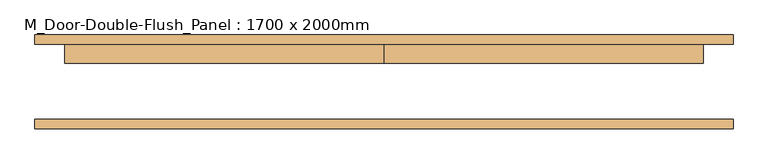
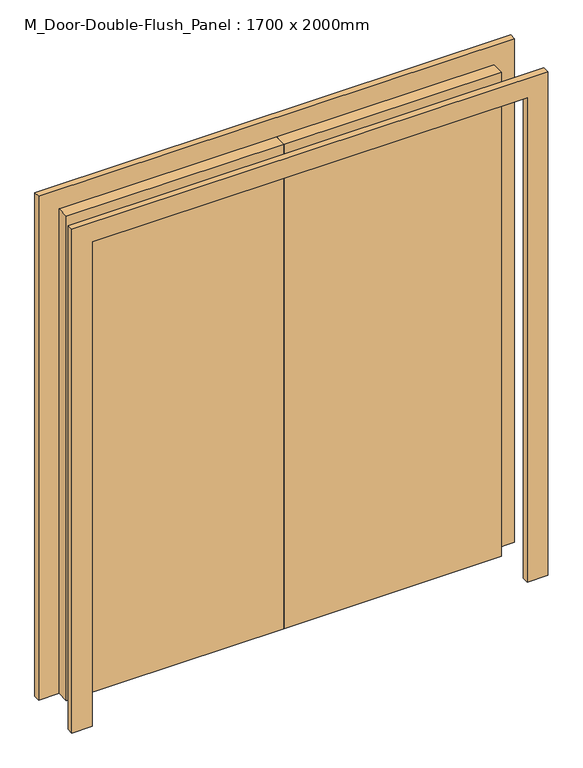
"""IFC4 building model written with IfcOpenShell, lengths in millimetres: door geometry, M_Door-Double-Flush_Panel : 1700 x 2000mm."""

from ifc_helpers import new_model, si_unit, frame, origin, origin_with_axes, place, context, project, spatial, polyline, outline, extrude, source, transform, mapped, element, save


def m_door_double_flush_panel_1700_x_2000mm_deeb3825(model_context):
    return source(origin(), model_context, "Body", "SweptSolid", [
        extrude(outline(polyline([(2000.0, -850.0), (2000.0, 850.0), (0.0, 850.0), (0.0, 930.0), (2080.0, 930.0), (2080.0, -930.0), (0.0, -930.0), (0.0, -850.0), (2000.0, -850.0)])), frame((0.0, -125.0, 0.0), z_axis=(0.0, 1.0, 0.0), x_axis=(0.0, 0.0, 1.0)), (0.0, 0.0, 1.0), 25.0),
        extrude(outline(polyline([(2000.0, -850.0), (2000.0, 850.0), (0.0, 850.0), (0.0, 930.0), (2080.0, 930.0), (2080.0, -930.0), (0.0, -930.0), (0.0, -850.0), (2000.0, -850.0)])), frame((0.0, 100.0, 0.0), z_axis=(0.0, 1.0, 0.0), x_axis=(0.0, 0.0, 1.0)), (0.0, 0.0, 1.0), 25.0),
        extrude(outline(polyline([(0.0, 100.0), (850.0, 100.0), (850.0, 50.0), (0.0, 50.0), (0.0, 100.0)])), origin_with_axes(), (0.0, 0.0, 1.0), 2000.0),
        extrude(outline(polyline([(-850.0, 100.0), (0.0, 100.0), (0.0, 50.0), (-850.0, 50.0), (-850.0, 100.0)])), origin_with_axes(), (0.0, 0.0, 1.0), 2000.0),
    ])


if __name__ == "__main__":
    model = new_model("IFC4")
    model_context = context("Model", 3, world=origin())
    ifc_project = project(units=[si_unit("LENGTHUNIT", "METRE", prefix="MILLI")], contexts=[model_context])
    site = spatial("IfcSite", under=ifc_project)
    building = spatial("IfcBuilding", under=site)
    placement = place(None, origin())
    m_door_double_flush_panel_1700_x_2000mm_shape = m_door_double_flush_panel_1700_x_2000mm_deeb3825(model_context)
    element("IfcDoor", 1, ObjectType="M_Door-Double-Flush_Panel : 1700 x 2000mm", at=placement, inside=building, context=model_context, shape_type="MappedRepresentation", body=[
        mapped(m_door_double_flush_panel_1700_x_2000mm_shape, transform((0.0, 0.0, 0.0), x_axis=(1.0, 0.0, 0.0), y_axis=(0.0, 1.0, 0.0), z_axis=(0.0, 0.0, 1.0))),
    ])
    save(model, "model.ifc")

# Revit data of these elements
# Type "M_Door-Double-Flush_Panel : 1700 x 2000mm"
#   Type Mark = "41"
#   Construction Type Id = "DOOR"
#   Assembly Code = "C1020"
#   Analytic Construction = "Wooden"
#   Thickness = 50 mm
#   Thermal Resistance (R) = 0.455703 (m²·K)/W
#   Swing Angle [instance default] = 90.00°
#   Panel Width = 850 mm
#   Heat Transfer Coefficient (U) = 2.19465 W/(m²·K)
#   Height = 2000 mm
#   Trim Projection Ext = 25 mm
#   Trim Projection Int = 25 mm
#   Trim Width = 80 mm
#   Width = 1700 mm
#   Panel Material = Wood - Birch - Solid Stained Light Low Gloss
#   Trim Material = Paint - Sienna
#   Visual Light Transmittance = 0
#   Solar Heat Gain Coefficient = 0
#   Function = (empty or 0)
#   Wall Closure = (empty or 0)
# Element 1 (IfcDoor, "M_Door-Double-Flush_Panel : 1700 x 2000mm")
#   Materials on its faces: "Paint - Sienna", "Wood - Birch - Solid Stained Light Low Gloss"
# Materials
#   "Wood - Birch - Solid Stained Light Low Gloss": class "Wood", colour RGB 210 159 95, transparency 0, Cost = 0
#   "Paint - Sienna": class "Miscellaneous", colour RGB 118 70 51, transparency 0, Cost = 0
